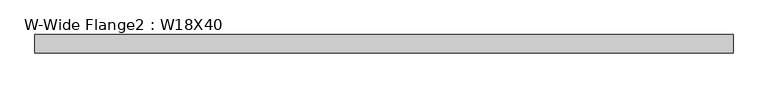
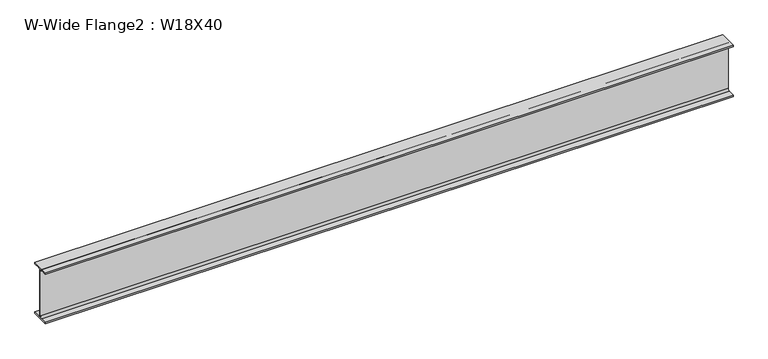
"""IFC4 building model written with IfcOpenShell, lengths in millimetres: beam geometry, W-Wide Flange2 : W18X40."""

from ifc_helpers import new_model, si_unit, point, frame, frame_2d, origin, place, context, project, spatial, polyline, circle_curve, trimmed, segment, composite_curve, outline, extrude, source, transform, mapped, element, save


def w_wide_flange2_w18x40_66fddd83(model_context):
    return source(origin(), model_context, "Body", "SweptSolid", [
        extrude(outline(composite_curve([segment(polyline([(76.454, -213.995), (76.454, -227.33), (-76.454, -227.33), (-76.454, -213.995), (-20.828, -213.995)]), True, "CONTINUOUS"), segment(trimmed(circle_curve(frame_2d((-20.828, -197.1675)), 16.8275), [point((-20.828, -213.995))], [point((-4.0005, -197.1675))], True, "CARTESIAN"), True, "CONTINUOUS"), segment(polyline([(-4.0005, -197.1675), (-4.0005, 197.1675)]), True, "CONTINUOUS"), segment(trimmed(circle_curve(frame_2d((-20.828, 197.1675)), 16.8275), [point((-4.0005, 197.1675))], [point((-20.828, 213.995))], True, "CARTESIAN"), True, "CONTINUOUS"), segment(polyline([(-20.828, 213.995), (-76.454, 213.995), (-76.454, 227.33), (76.454, 227.33), (76.454, 213.995), (20.828, 213.995)]), True, "CONTINUOUS"), segment(trimmed(circle_curve(frame_2d((20.828, 197.1675)), 16.8275), [point((20.828, 213.995))], [point((4.0005, 197.1675))], True, "CARTESIAN"), True, "CONTINUOUS"), segment(polyline([(4.0005, 197.1675), (4.0005, -197.1675)]), True, "CONTINUOUS"), segment(trimmed(circle_curve(frame_2d((20.828, -197.1675)), 16.8275), [point((4.0005, -197.1675))], [point((20.828, -213.995))], True, "CARTESIAN"), True, "CONTINUOUS"), segment(polyline([(20.828, -213.995), (76.454, -213.995)]), True, "CONTINUOUS")], self_intersect=False)), frame((-2881.3125, 0.0, 0.0), z_axis=(1.0, 0.0, 0.0), x_axis=(0.0, 1.0, 0.0)), (0.0, 0.0, 1.0), 5757.465625),
    ])


if __name__ == "__main__":
    model = new_model("IFC4")
    model_context = context("Model", 3, world=origin())
    ifc_project = project(units=[si_unit("LENGTHUNIT", "METRE", prefix="MILLI")], contexts=[model_context])
    site = spatial("IfcSite", under=ifc_project)
    building = spatial("IfcBuilding", under=site)
    placement = place(None, origin())
    w_wide_flange2_w18x40_shape = w_wide_flange2_w18x40_66fddd83(model_context)
    element("IfcBeam", 1, ObjectType="W-Wide Flange2 : W18X40", at=placement, inside=building, context=model_context, shape_type="MappedRepresentation", body=[
        mapped(w_wide_flange2_w18x40_shape, transform((0.0, 0.0, 0.0), x_axis=(1.0, 0.0, 0.0), y_axis=(0.0, 1.0, 0.0), z_axis=(0.0, 0.0, 1.0))),
    ])
    save(model, "model.ifc")

# Revit data of these elements
# Type "W-Wide Flange2 : W18X40"
#   Assembly Code = "B10"
#   W = 40
#   Length [instance default] = 5' - 0"
#   bf = 0' - 6.02"
#   d = 1' - 5.9"
#   k = 0' - 1 3/16"
#   k2 = 0' - 0.6625"
#   tf = 0' - 0.525"
#   tw = 0' - 0.315"
#   A = 0.0819444 SF
#   Structural Material [instance default] = Steel ASTM A992
# Element 1 (IfcBeam, "W-Wide Flange2 : W18X40")
#   Materials on its faces: "Steel ASTM A992"
# Materials
#   "Steel ASTM A992": class "Metal", colour RGB 199 199 199, transparency 0, Description = "Structural steel 50ksi", Cost = 0
